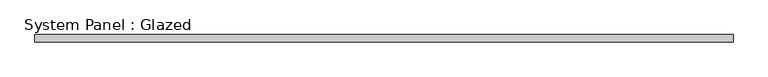
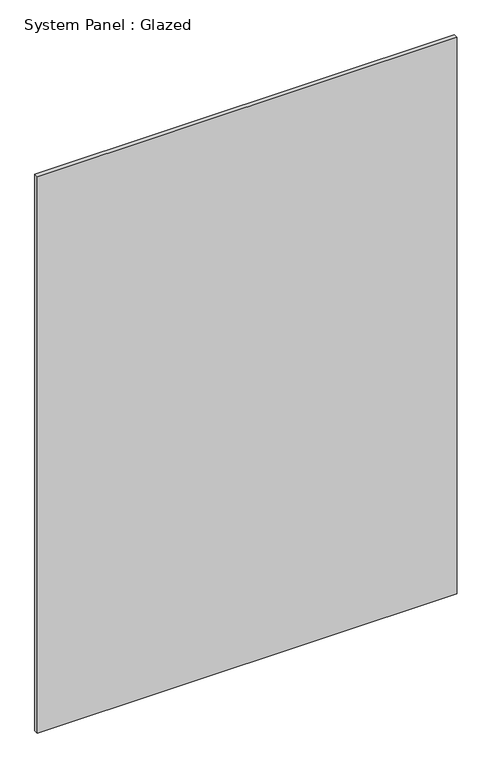
"""IFC4 building model written with IfcOpenShell, lengths in millimetres: plate geometry, System Panel : Glazed."""

from ifc_helpers import new_model, si_unit, origin, origin_with_axes, place, context, project, spatial, polyline, outline, extrude, source, transform, mapped, element, save


def system_panel_glazed_ce7d9ee4(model_context):
    return source(origin(), model_context, "Body", "SweptSolid", [
        extrude(outline(polyline([(1202.784159, 24.5), (-1202.784159, 24.5), (-1202.784159, 49.5), (1202.784159, 49.5), (1202.784159, 24.5)])), origin_with_axes(), (0.0, 0.0, 1.0), 3370.0),
    ])


if __name__ == "__main__":
    model = new_model("IFC4")
    model_context = context("Model", 3, world=origin())
    ifc_project = project(units=[si_unit("LENGTHUNIT", "METRE", prefix="MILLI")], contexts=[model_context])
    site = spatial("IfcSite", under=ifc_project)
    building = spatial("IfcBuilding", under=site)
    placement = place(None, origin())
    system_panel_glazed_shape = system_panel_glazed_ce7d9ee4(model_context)
    element("IfcPlate", 1, ObjectType="System Panel : Glazed", at=placement, inside=building, context=model_context, shape_type="MappedRepresentation", body=[
        mapped(system_panel_glazed_shape, transform((0.0, 0.0, 0.0), x_axis=(1.0, 0.0, 0.0), y_axis=(0.0, 1.0, 0.0), z_axis=(0.0, 0.0, 1.0))),
    ])
    save(model, "model.ifc")

# Revit data of these elements
# Type "System Panel : Glazed"
#   Construction Type Id = "GSP4R"
#   Analytic Construction = "1/8 in Pilkington single glazing"
#   Visual Light Transmittance = 0.9
#   Solar Heat Gain Coefficient = 0.86
#   Heat Transfer Coefficient (U) = 6.7069 W/(m²·K)
#   Define Thermal Properties by = 1
# Element 1 (IfcPlate, "System Panel : Glazed")
#   Materials on its faces: "Glass"
# Materials
#   "Glass": class "Glass", colour RGB 245 245 243, transparency 1, Description = "Soda Lime Glass", Cost = 0
